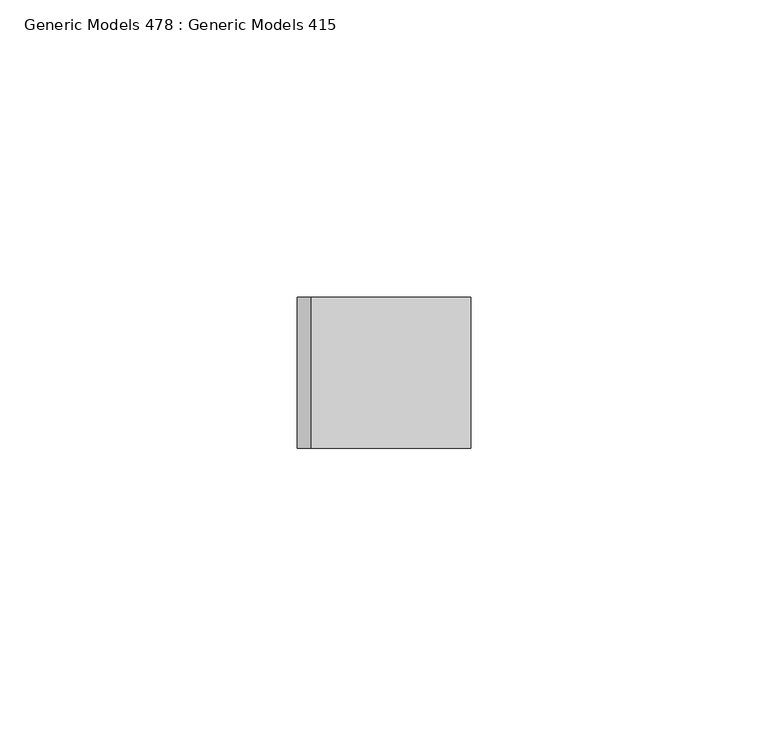
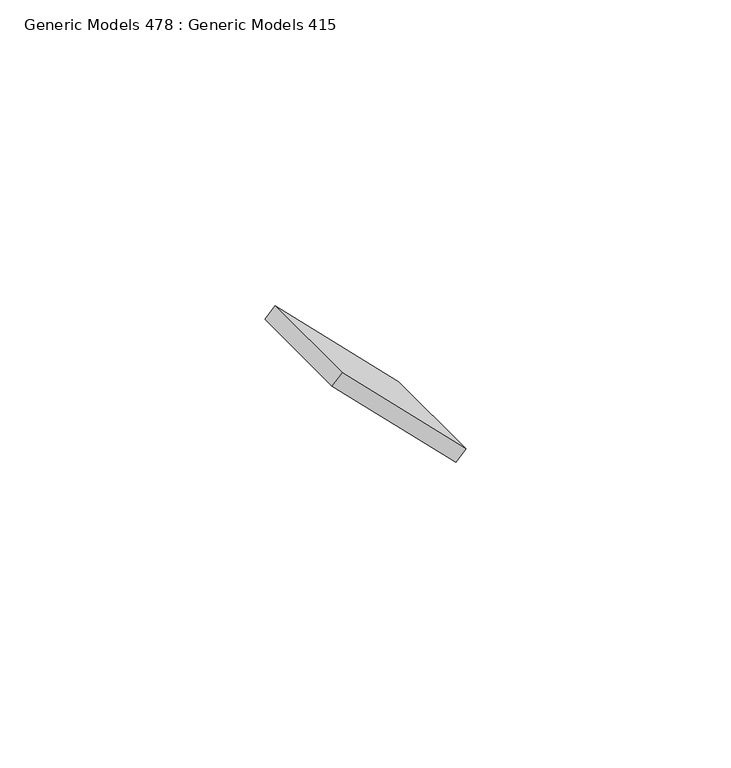
"""IFC4 building model written with IfcOpenShell, lengths in millimetres: proxy geometry, Generic Models 478 : Generic Models 415."""

from ifc_helpers import new_model, si_unit, frame, origin, place, context, project, spatial, polyline, outline, extrude, source, transform, mapped, element, save


def generic_models_478_generic_models_415_85b6ebb1(model_context):
    return source(origin(), model_context, "Body", "SweptSolid", [
        extrude(outline(polyline([(0.0, -38.1), (0.0, 0.0), (25.4, 0.0), (25.4, -38.1), (0.0, -38.1)])), frame((-6869.8996186, -4475.9863946, 127908.5002957), z_axis=(0.7071067811864907, 0.0, 0.7071067811866044), x_axis=(0.0, -1.0, 0.0)), (0.0, 0.0, 1.0), 3.175),
    ])


if __name__ == "__main__":
    model = new_model("IFC4")
    model_context = context("Model", 3, world=origin())
    ifc_project = project(units=[si_unit("LENGTHUNIT", "METRE", prefix="MILLI")], contexts=[model_context])
    site = spatial("IfcSite", under=ifc_project)
    building = spatial("IfcBuilding", under=site)
    placement = place(None, origin())
    generic_models_478_generic_models_415_shape = generic_models_478_generic_models_415_85b6ebb1(model_context)
    element("IfcBuildingElementProxy", 1, Name="Generic Models 478 : Generic Models 415", ObjectType="Generic Models 478 : Generic Models 415", at=placement, inside=building, context=model_context, shape_type="MappedRepresentation", body=[
        mapped(generic_models_478_generic_models_415_shape, transform((0.0, 0.0, 0.0), x_axis=(1.0, 0.0, 0.0), y_axis=(0.0, 1.0, 0.0), z_axis=(0.0, 0.0, 1.0))),
    ])
    save(model, "model.ifc")

# Revit data of these elements
# Element 1 (IfcBuildingElementProxy, "Generic Models 478 : Generic Models 415")
#   Materials on its faces: "_WELDED STEEL TABS FOR LOUVER ATTACHMENT"
# Materials
#   "_WELDED STEEL TABS FOR LOUVER ATTACHMENT": class "Metal", colour RGB 199 199 199, transparency 0, Description = "Structural steel 50ksi", Cost = 0
